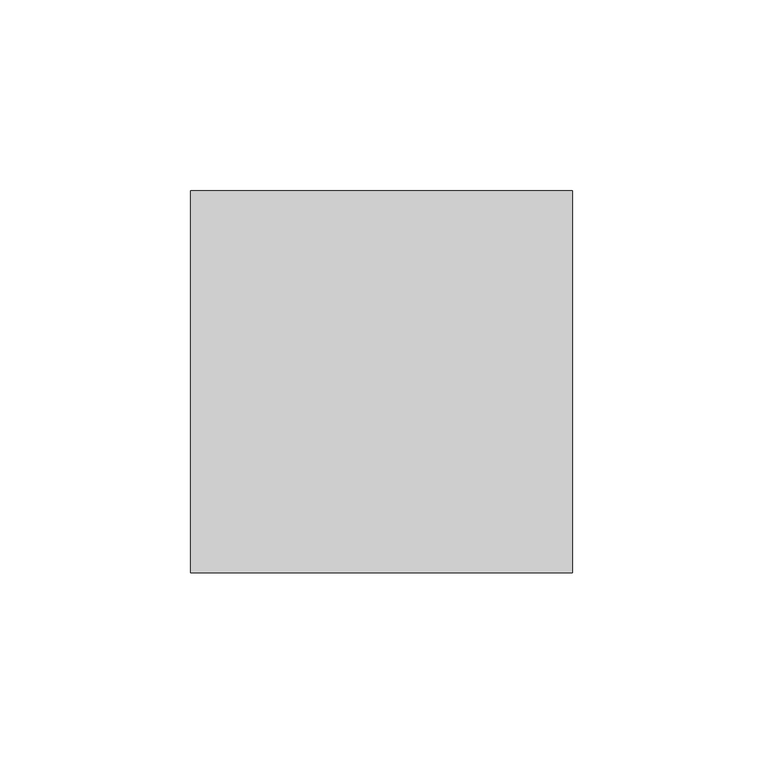
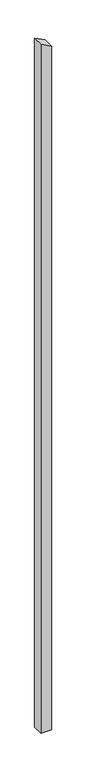
"""IFC4 building model written with IfcOpenShell, lengths in millimetres: column geometry, Holzstütze 159006 : Holzstütze 159006."""

from ifc_helpers import new_model, si_unit, frame, origin, place, context, project, spatial, polyline, outline, extrude, source, transform, mapped, element, save


def column_1fc37466(model_context):
    return source(origin(), model_context, "Body", "SweptSolid", [
        extrude(outline(polyline([(-500.0, 174197.7593015), (-500.0, 174297.7593015), (6345.7118258, 174297.7593015), (6396.6643707, 174197.7593015), (-500.0, 174197.7593015)])), frame((0.0, 47884.7962965, 0.0), z_axis=(0.0, 1.0, 0.0), x_axis=(0.0, 0.0, 1.0)), (0.0, 0.0, 1.0), 100.0),
    ])


if __name__ == "__main__":
    model = new_model("IFC4")
    model_context = context("Model", 3, world=origin())
    ifc_project = project(units=[si_unit("LENGTHUNIT", "METRE", prefix="MILLI")], contexts=[model_context])
    site = spatial("IfcSite", under=ifc_project)
    building = spatial("IfcBuilding", under=site)
    placement = place(None, origin())
    column_shape = column_1fc37466(model_context)
    element("IfcColumn", 1, ObjectType="Holzstütze 159006 : Holzstütze 159006", at=placement, inside=building, context=model_context, shape_type="MappedRepresentation", body=[
        mapped(column_shape, transform((0.0, 0.0, 0.0), x_axis=(1.0, 0.0, 0.0), y_axis=(0.0, 1.0, 0.0), z_axis=(0.0, 0.0, 1.0))),
    ])
    save(model, "model.ifc")

# Revit data of these elements
# Type "Holzstütze 159006 : Holzstütze 159006"
#   Abrechnungsart = "m"
#   Allright_Bauteil_ID = "0152St 0000143382"
#   Bezeichnung = "Holzstütze"
#   Codetext = "ST-HOLZ\\"
#   Gewerk = "Zimmer- und Holzbauarbeiten"
#   Material = "Holz"
#   Objektname = "Stütze"
#   NameOverride = "Holzstütze"
#   Reference = "Holzstütze"
#   Status = "NEW"
#   ThermalTransmittance = 0.0000 BTU/(h·ft²·°F)
#   Roll = 0.00°
#   Slope = 0.00°
#   2D Interaktion = yes
#   IsExternal = yes
#   LoadBearing = yes
# Element 1 (IfcColumn, "Holzstütze 159006 : Holzstütze 159006")
#   Materials on its faces: "holzschalung"
# Materials
#   "holzschalung": class "Unassigned", colour RGB 128 128 128, transparency 0
